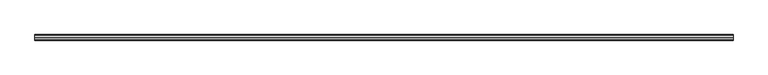
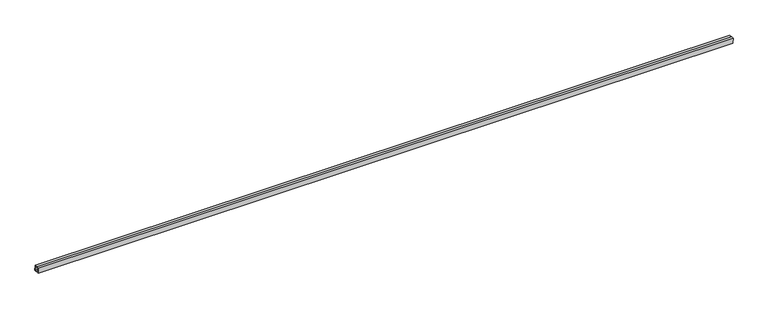
"""IFC4 building model written with IfcOpenShell, lengths in millimetres: proxy geometry, Inner panel:Inner panel:1:Inner panel:1 : Inner panel:Inner panel:300324:2:Inner panel:1:Inner panel:1 : Inner panel:Inner panel:300324:2 : Inner panel:Inner panel:1:Inner panel:1 : Inner panel:Inner panel:300324:300043:45 : Inner panel:Inner panel:1:Inner panel:1 : Inner panel:Inner panel:300324:2:Inner panel:1:Inner panel:1 : Inner panel:Inner panel:300324:2 : Inner panel:Inner panel:1:Inner panel:1 : Inner panel:Inner panel:300324:300043:308120."""

from ifc_helpers import new_model, si_unit, frame, origin, place, context, project, spatial, polyline, outline, extrude, source, transform, mapped, element, save


def generic_models_cff6365f(model_context):
    return source(origin(), model_context, "Body", "SweptSolid", [
        extrude(outline(polyline([(-578476.5317668, 3971.7383355), (-578458.2913437, 3972.4983531), (-578456.7052199, 3934.431383), (-578494.77219, 3932.8452593), (-578496.3583138, 3970.9122294), (-578478.1178906, 3971.672247), (-578478.0187579, 3969.2930614), (-578493.8799954, 3968.6321765), (-578492.4921371, 3935.3235776), (-578459.1835383, 3936.7114359), (-578460.5713966, 3970.0200347), (-578476.4326341, 3969.3591498), (-578476.5317668, 3971.7383355)])), frame((607854.1367239, 0.0, 0.0), z_axis=(1.0, 0.0, 0.0), x_axis=(0.0, 1.0, 0.0)), (0.0, 0.0, 1.0), 4876.8),
    ])


if __name__ == "__main__":
    model = new_model("IFC4")
    model_context = context("Model", 3, world=origin())
    ifc_project = project(units=[si_unit("LENGTHUNIT", "METRE", prefix="MILLI")], contexts=[model_context])
    site = spatial("IfcSite", under=ifc_project)
    building = spatial("IfcBuilding", under=site)
    placement = place(None, origin())
    generic_models_shape = generic_models_cff6365f(model_context)
    element("IfcBuildingElementProxy", 1, Name="Inner panel:Inner panel:1:Inner panel:1 : Inner panel:Inner panel:300324:2:Inner panel:1:Inner panel:1 : Inner panel:Inner panel:300324:2 : Inner panel:Inner panel:1:Inner panel:1 : Inner panel:Inner panel:300324:300043:45 : Inner panel:Inner panel:1:Inner panel:1 : Inner panel:Inner panel:300324:2:Inner panel:1:Inner panel:1 : Inner panel:Inner panel:300324:2 : Inner panel:Inner panel:1:Inner panel:1 : Inner panel:Inner panel:300324:300043:308120", ObjectType="Inner panel:Inner panel:1:Inner panel:1 : Inner panel:Inner panel:300324:2:Inner panel:1:Inner panel:1 : Inner panel:Inner panel:300324:2 : Inner panel:Inner panel:1:Inner panel:1 : Inner panel:Inner panel:300324:300043:45 : Inner panel:Inner panel:1:Inner panel:1 : Inner panel:Inner panel:300324:2:Inner panel:1:Inner panel:1 : Inner panel:Inner panel:300324:2 : Inner panel:Inner panel:1:Inner panel:1 : Inner panel:Inner panel:300324:300043:308120", at=placement, inside=building, context=model_context, shape_type="MappedRepresentation", body=[
        mapped(generic_models_shape, transform((0.0, 0.0, 0.0), x_axis=(1.0, 0.0, 0.0), y_axis=(0.0, 1.0, 0.0), z_axis=(0.0, 0.0, 1.0))),
    ])
    save(model, "model.ifc")

# Revit data of these elements
# Type "Inner panel:Inner panel:1:Inner panel:1 : Inner panel:Inner panel:300324:2:Inner panel:1:Inner panel:1 : Inner panel:Inner panel:300324:2 : Inner panel:Inner panel:1:Inner panel:1 : Inner panel:Inner panel:300324:300043:45 : Inner panel:Inner panel:1:Inner panel:1 : Inner panel:Inner panel:300324:2:Inner panel:1:Inner panel:1 : Inner panel:Inner panel:300324:2 : Inner panel:Inner panel:1:Inner panel:1 : Inner panel:Inner panel:300324:300043:308120"
#   NameOverride = "Inner panel:Inner panel:1:Inner panel:1 : Inner panel:Inner panel:300324:2:Inner panel:1:Inner panel:1 : Inner panel:Inner panel:300324:2 : Inner panel:Inner panel:1:Inner panel:1 : Inner panel:Inner panel:300324:300043:308120"
#   ObjectTypeOverride = "Inner panel:1:Inner panel:1 : Inner panel:Inner panel:300324:2 : Inner panel:Inner panel:1:Inner panel:1 : Inner panel:Inner panel:300324:300043"
#   Reference = "Inner panel"
#   Tag = "308120"
# Element 1 (IfcBuildingElementProxy, "Inner panel:Inner panel:1:Inner panel:1 : Inner panel:Inner panel:300324:2:Inner panel:1:Inner panel:1 : Inner panel:Inner panel:300324:2 : Inner panel:Inner panel:1:Inner panel:1 : Inner panel:Inner panel:300324:300043:45 : Inner panel:Inner panel:1:Inner panel:1 : Inner panel:Inner panel:300324:2:Inner panel:1:Inner panel:1 : Inner panel:Inner panel:300324:2 : Inner panel:Inner panel:1:Inner panel:1 : Inner panel:Inner panel:300324:300043:308120")
#   Materials on its faces: "1 1/2\" X 1 1/2\" SPLIT-SEAM SQUARE TUBING (~24\" CANTILEVER FROM C.L. OF GLULAM)"
# Materials
#   "1 1/2\" X 1 1/2\" SPLIT-SEAM SQUARE TUBING (~24\" CANTILEVER FROM C.L. OF GLULAM)": class "Unassigned", colour RGB 202 201 200, transparency 0, Cost = 0
